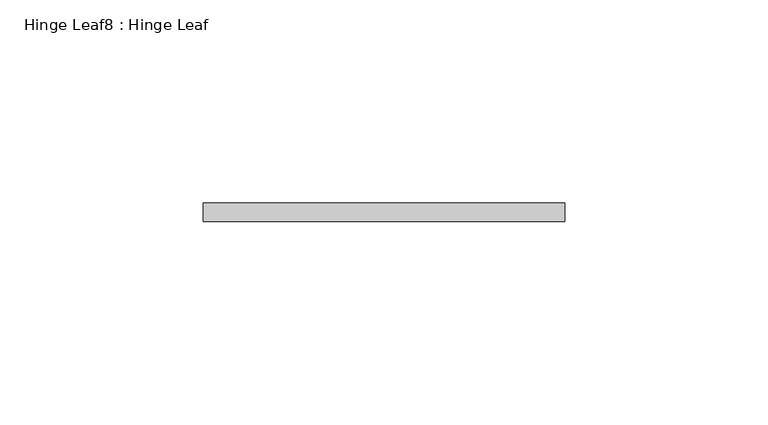
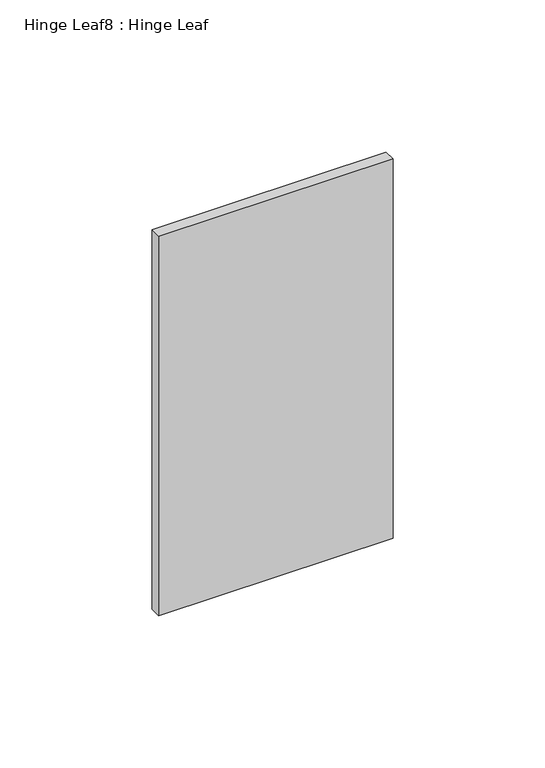
"""IFC4 building model written with IfcOpenShell, lengths in millimetres: proxy geometry, Hinge Leaf8 : Hinge Leaf."""

from ifc_helpers import new_model, si_unit, frame, origin, place, context, project, spatial, polyline, outline, extrude, source, transform, mapped, element, save


def hinge_leaf8_hinge_leaf_946f20d6(model_context):
    return source(origin(), model_context, "Body", "SweptSolid", [
        extrude(outline(polyline([(587327.7934739, -533980.5883841), (587327.7934739, -533976.0163841), (587416.6934739, -533976.0163841), (587416.6934739, -533980.5883841), (587327.7934739, -533980.5883841)])), frame((0.0, 0.0, 1936.75), z_axis=(0.0, 0.0, 1.0), x_axis=(1.0, 0.0, 0.0)), (0.0, 0.0, 1.0), 152.4),
    ])


if __name__ == "__main__":
    model = new_model("IFC4")
    model_context = context("Model", 3, world=origin())
    ifc_project = project(units=[si_unit("LENGTHUNIT", "METRE", prefix="MILLI")], contexts=[model_context])
    site = spatial("IfcSite", under=ifc_project)
    building = spatial("IfcBuilding", under=site)
    placement = place(None, origin())
    hinge_leaf8_hinge_leaf_shape = hinge_leaf8_hinge_leaf_946f20d6(model_context)
    element("IfcBuildingElementProxy", 1, Name="Hinge Leaf8 : Hinge Leaf", ObjectType="Hinge Leaf8 : Hinge Leaf", at=placement, inside=building, context=model_context, shape_type="MappedRepresentation", body=[
        mapped(hinge_leaf8_hinge_leaf_shape, transform((0.0, 0.0, 0.0), x_axis=(1.0, 0.0, 0.0), y_axis=(0.0, 1.0, 0.0), z_axis=(0.0, 0.0, 1.0))),
    ])
    save(model, "model.ifc")

# Revit data of these elements
# Element 1 (IfcBuildingElementProxy, "Hinge Leaf8 : Hinge Leaf")
#   Materials on its faces: "6\"X6\" WELD-ON STL BUTT HINGE"
# Materials
#   "6\"X6\" WELD-ON STL BUTT HINGE": class "Metal", colour RGB 189 187 185, transparency 0, Description = "Carbon steel", Cost = 0
